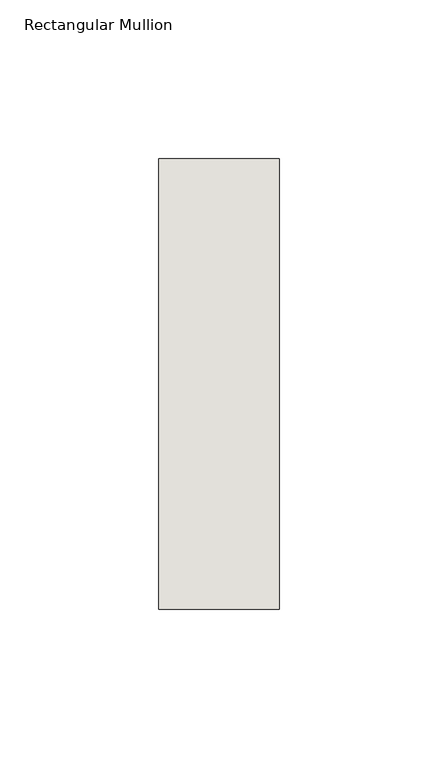
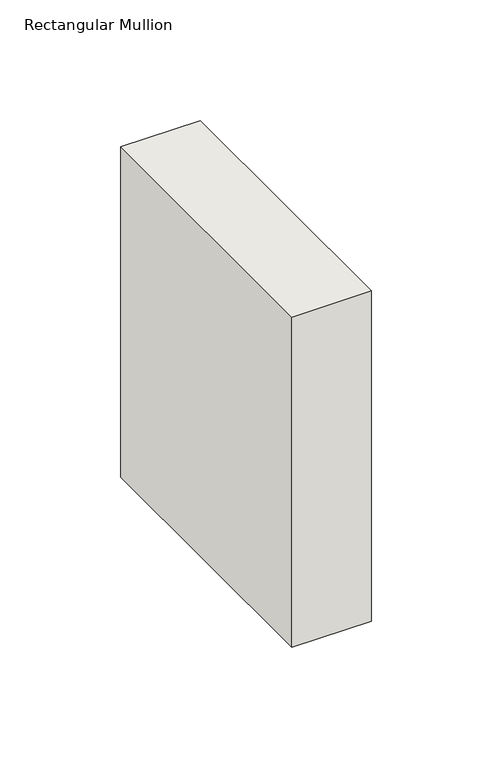
"""IFC4 building model written with IfcOpenShell, lengths in millimetres: wall geometry, Rectangular Mullion : NLRS_21_CWM_hsb-regel 38x142_gen_rsf."""

from ifc_helpers import new_model, si_unit, frame, origin, place, context, project, spatial, polyline, outline, extrude, source, transform, mapped, element, save


def rectangular_mullion_c6f7c22d(model_context):
    return source(origin(), model_context, "Body", "SweptSolid", [
        extrude(outline(polyline([(-38.0, -71.0), (-38.0, 71.0), (0.0, 71.0), (0.0, -71.0), (-38.0, -71.0)])), frame((0.0, 0.0, -167.1558939), z_axis=(0.0, 0.0, 1.0), x_axis=(1.0, 0.0, 0.0)), (0.0, 0.0, 1.0), 167.1558939),
    ])


if __name__ == "__main__":
    model = new_model("IFC4")
    model_context = context("Model", 3, world=origin())
    ifc_project = project(units=[si_unit("LENGTHUNIT", "METRE", prefix="MILLI")], contexts=[model_context])
    site = spatial("IfcSite", under=ifc_project)
    building = spatial("IfcBuilding", under=site)
    placement = place(None, origin())
    rectangular_mullion_shape = rectangular_mullion_c6f7c22d(model_context)
    element("IfcWall", 1, ObjectType="Rectangular Mullion : NLRS_21_CWM_hsb-regel 38x142_gen_rsf", at=placement, inside=building, context=model_context, shape_type="MappedRepresentation", body=[
        mapped(rectangular_mullion_shape, transform((0.0, 0.0, 0.0), x_axis=(1.0, 0.0, 0.0), y_axis=(0.0, 1.0, 0.0), z_axis=(0.0, 0.0, 1.0))),
    ])
    save(model, "model.ifc")

# Revit data of these elements
# Type "Rectangular Mullion : NLRS_21_CWM_hsb-regel 38x142_gen_rsf"
#   Type IfcGUID = "07M7mRoiH1CR8m_RSKIwpF"
#   Assembly Code = "21.10"
#   IfcExportAs = "IfcWall"
#   built-in parameter 1007322 = 0.465879 (stored number, unit not read)
#   built-in parameter 1007321 = 0.062336 (stored number, unit not read)
#   built-in parameter 1007320 = 0.062336 (stored number, unit not read)
# Element 1 (IfcWall, "Rectangular Mullion : NLRS_21_CWM_hsb-regel 38x142_gen_rsf")
#   Materials on its faces: "NLRS_i2_hout naaldhout vuren_gen_rsf"
# Materials
#   "NLRS_i2_hout naaldhout vuren_gen_rsf": class "I - Hout", colour RGB 234 199 147, transparency 0, Keynote = "i2", Manufacturer = "Revit Standards Foundation", URL = "www.revitstandards.org", Description = "hout vuren", Cost = 0
